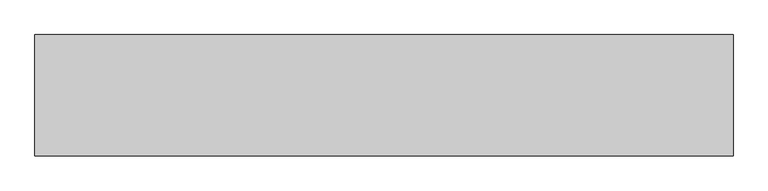
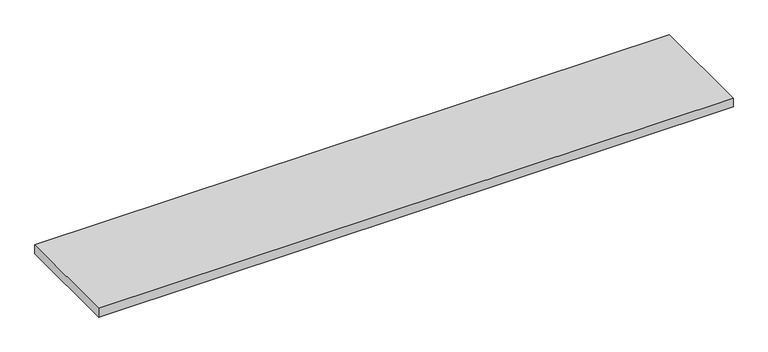
"""IFC4 building model written with IfcOpenShell, lengths in millimetres: furniture geometry, OD_CW_Closet : OD_CW_Closet."""

from ifc_helpers import new_model, si_unit, frame, origin, place, context, project, spatial, polyline, outline, extrude, source, transform, mapped, element, save


def furniture_88d1f670(model_context):
    return source(origin(), model_context, "Body", "SweptSolid", [
        extrude(outline(polyline([(18.7377049, -609.6), (18.7377049, 0.0), (3519.1752049, 0.0), (3519.1752049, -609.6), (18.7377049, -609.6)])), frame((0.0, 0.0, 1828.8), z_axis=(0.0, 0.0, 1.0), x_axis=(1.0, 0.0, 0.0)), (0.0, 0.0, 1.0), 50.8),
    ])


if __name__ == "__main__":
    model = new_model("IFC4")
    model_context = context("Model", 3, world=origin())
    ifc_project = project(units=[si_unit("LENGTHUNIT", "METRE", prefix="MILLI")], contexts=[model_context])
    site = spatial("IfcSite", under=ifc_project)
    building = spatial("IfcBuilding", under=site)
    placement = place(None, origin())
    furniture_shape = furniture_88d1f670(model_context)
    element("IfcFurniture", 1, ObjectType="OD_CW_Closet : OD_CW_Closet", at=placement, inside=building, context=model_context, shape_type="MappedRepresentation", body=[
        mapped(furniture_shape, transform((0.0, 0.0, 0.0), x_axis=(1.0, 0.0, 0.0), y_axis=(0.0, 1.0, 0.0), z_axis=(0.0, 0.0, 1.0))),
    ])
    save(model, "model.ifc")

# Revit data of these elements
# Type "OD_CW_Closet : OD_CW_Closet"
#   OD_CW_Width [instance default] = 2' - 9"
#   OD_CW_Off Floor [instance default] = 6' - 0"
#   OD_CW_Length [instance default] = 6' - 9"
#   OD_CW_Height [instance default] = 0' - 2"
#   Depth = 2' - 0"
#   Height = 3' - 0"
#   Width = 4' - 0"
#   OD_CW_Material_Countertop [instance default] = none
# Element 1 (IfcFurniture, "OD_CW_Closet : OD_CW_Closet")
#   OD_CW_Width = 2' - 0"
#   OD_CW_Length = 11' - 5 13/16"
#   Materials on its faces: "CASEWORK"
# Materials
#   "CASEWORK": class "Generic", colour RGB 181 181 181, transparency 0, Cost = 0
